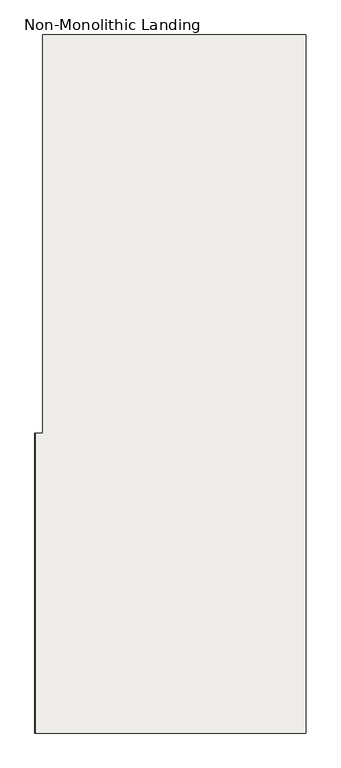
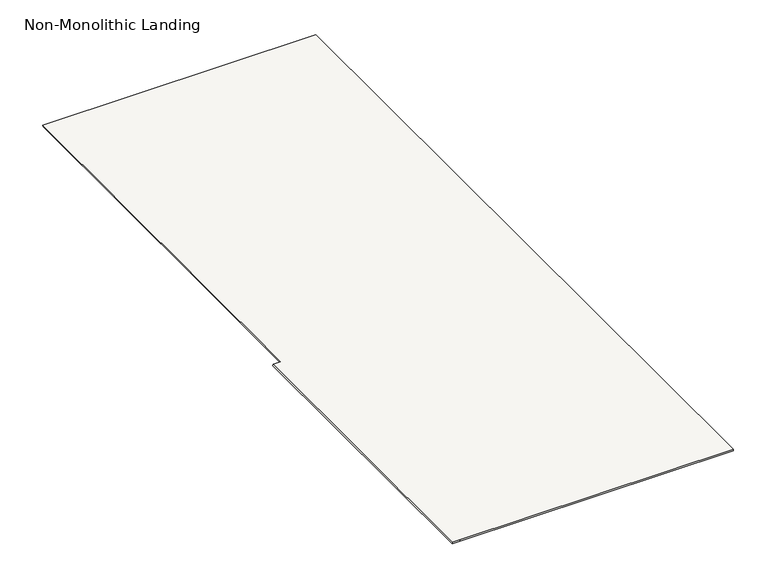
"""IFC4 building model written with IfcOpenShell, lengths in millimetres: slab geometry, Non-Monolithic Landing."""

from ifc_helpers import new_model, si_unit, origin, place, context, project, spatial, faceted_brep, source, transform, mapped, element, save


def non_monolithic_landing_6458ee0e(model_context):
    return source(origin(), model_context, "Body", "Brep", [
        faceted_brep([(-13356.0590357, 11470.4345331, 4088.8888889), (-13356.9027857, 11470.4345331, 4082.8888889), (-13356.9027857, 10220.4345331, 4082.8888889), (-13356.0590357, 10220.4345331, 4088.8888889), (-13325.0, 12030.4345331, 4088.8888889), (-13325.0, 11470.4345331, 4088.8888889), (-13325.0, 10220.4345331, 4088.8888889), (-12225.0, 10220.4345331, 4088.8888889), (-12225.0, 13130.4345331, 4088.8888889), (-13325.0, 13130.4345331, 4088.8888889), (-13325.0, 11470.4345331, 4082.8888889), (-13325.0, 12030.4345331, 4082.8888889), (-13324.15625, 12030.4345331, 4082.8888889), (-13324.15625, 13130.4345331, 4082.8888889), (-12225.0, 13130.4345331, 4082.8888889), (-12225.0, 10220.4345331, 4082.8888889), (-13325.0, 10220.4345331, 4082.8888889)], [[[0, 1, 2, 3]], [[4, 5, 0, 3, 6, 7, 8, 9]], [[10, 11, 12, 13, 14, 15, 16, 2, 1]], [[5, 4, 11, 10]], [[0, 5, 10, 1]], [[6, 3, 2, 16]], [[7, 6, 16, 15]], [[8, 7, 15, 14]], [[9, 8, 14, 13]], [[4, 12, 11]], [[12, 4, 9, 13]]]),
    ])


if __name__ == "__main__":
    model = new_model("IFC4")
    model_context = context("Model", 3, world=origin())
    ifc_project = project(units=[si_unit("LENGTHUNIT", "METRE", prefix="MILLI")], contexts=[model_context])
    site = spatial("IfcSite", under=ifc_project)
    building = spatial("IfcBuilding", under=site)
    placement = place(None, origin())
    non_monolithic_landing_shape = non_monolithic_landing_6458ee0e(model_context)
    element("IfcSlab", 1, ObjectType="Non-Monolithic Landing", at=placement, inside=building, context=model_context, shape_type="MappedRepresentation", body=[
        mapped(non_monolithic_landing_shape, transform((0.0, 0.0, 0.0), x_axis=(1.0, 0.0, 0.0), y_axis=(0.0, 1.0, 0.0), z_axis=(0.0, 0.0, 1.0))),
    ])
    save(model, "model.ifc")

# Revit data of these elements
# Element 1 (IfcSlab, "Non-Monolithic Landing")
#   Materials on its faces: "Steel, Paint Finish, Dark Gray"
# Materials
#   "Steel, Paint Finish, Dark Gray": class "Metal", colour RGB 89 89 89, transparency 0, Description = "Steel, paint finish, dark gray, glossy", Cost = 0
